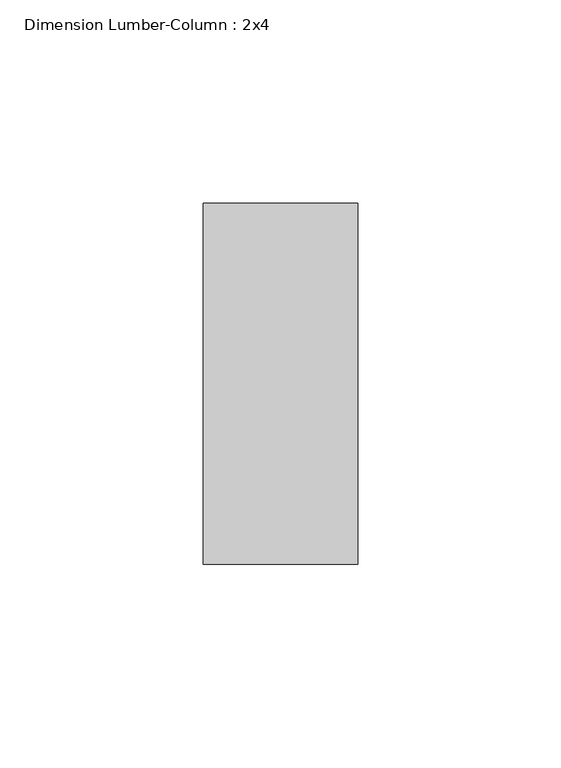
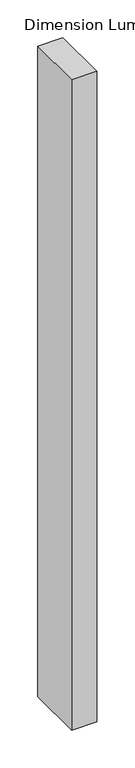
"""IFC4 building model written with IfcOpenShell, lengths in millimetres: column geometry, Dimension Lumber-Column : 2x4."""

from ifc_helpers import new_model, si_unit, frame, origin, place, context, project, spatial, polyline, outline, extrude, source, transform, mapped, element, save


def dimension_lumber_column_2x4_e2d4624f(model_context):
    return source(origin(), model_context, "Body", "SweptSolid", [
        extrude(outline(polyline([(19.05, 44.45), (19.05, -44.45), (-19.05, -44.45), (-19.05, 44.45), (19.05, 44.45)])), frame((0.0, 0.0, 56.35625), z_axis=(0.0, 0.0, 1.0), x_axis=(1.0, 0.0, 0.0)), (0.0, 0.0, 1.0), 1047.353125),
    ])


if __name__ == "__main__":
    model = new_model("IFC4")
    model_context = context("Model", 3, world=origin())
    ifc_project = project(units=[si_unit("LENGTHUNIT", "METRE", prefix="MILLI")], contexts=[model_context])
    site = spatial("IfcSite", under=ifc_project)
    building = spatial("IfcBuilding", under=site)
    placement = place(None, origin())
    dimension_lumber_column_2x4_shape = dimension_lumber_column_2x4_e2d4624f(model_context)
    element("IfcColumn", 1, ObjectType="Dimension Lumber-Column : 2x4", at=placement, inside=building, context=model_context, shape_type="MappedRepresentation", body=[
        mapped(dimension_lumber_column_2x4_shape, transform((0.0, 0.0, 0.0), x_axis=(1.0, 0.0, 0.0), y_axis=(0.0, 1.0, 0.0), z_axis=(0.0, 0.0, 1.0))),
    ])
    save(model, "model.ifc")

# Revit data of these elements
# Type "Dimension Lumber-Column : 2x4"
#   Int Type = "Interior"
#   Assembly Code = "B10"
#   Cost = 8.05
#   A = 0.0364583 SF
#   b = 0' - 1 1/2"
#   d = 0' - 3 1/2"
#   Structural Material [instance default] = Softwood, Lumber
# Element 1 (IfcColumn, "Dimension Lumber-Column : 2x4")
#   Structural Material = Douglas Fir #2
#   Materials on its faces: "Douglas Fir #2"
# Materials
#   "Softwood, Lumber": class "Wood", colour RGB 223 192 134, transparency 0, Description = "Pinus Echinata", Cost = 0
#   "Douglas Fir #2": class "Wood", colour RGB 223 192 134, transparency 0, Description = "Pinus Echinata", Cost = 0
